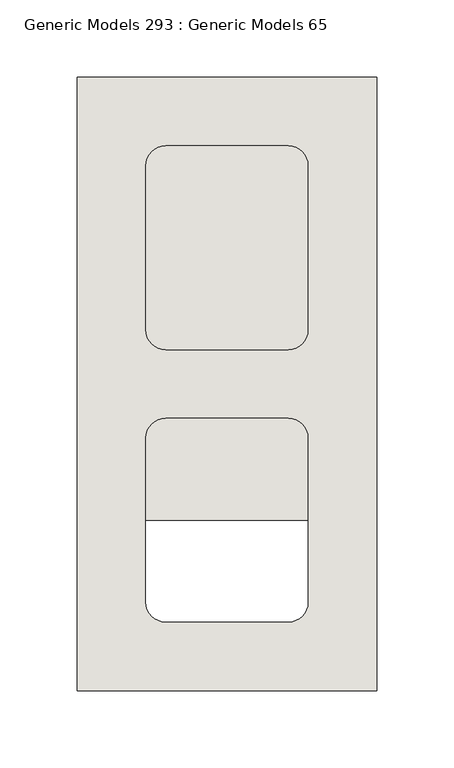
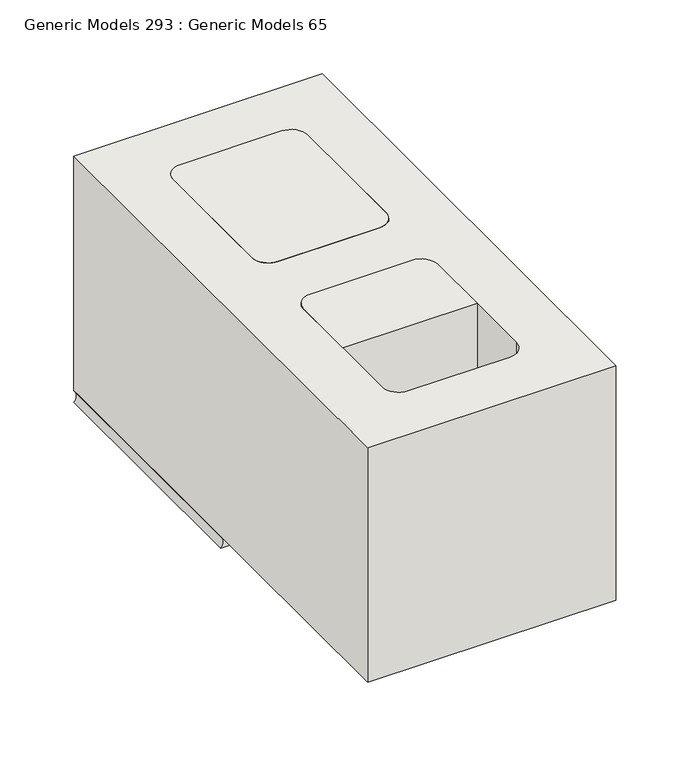
"""IFC4 building model written with IfcOpenShell, lengths in millimetres: wall geometry, Generic Models 293 : Generic Models 65."""

from ifc_helpers import new_model, si_unit, point, frame, frame_2d, origin, place, context, project, spatial, polyline, circle_curve, trimmed, segment, composite_curve, outline, extrude, source, transform, mapped, element, save
from ifc_brep_helpers import plane_surface, revolved_surface, advanced_brep


def generic_models_293_generic_models_65_16f1c2ea(model_context):
    return source(origin(), model_context, "Body", "SolidModel", [
        advanced_brep(
        [(430198.2125, 503.2375, 212.725), (430004.5375, 503.2375, 212.725), (430004.5375, 503.2375, 203.2), (430198.2125, 503.2375, 203.2), (430198.2125, 701.675, 212.725), (430198.2125, 701.675, 203.2), (430004.5375, 701.675, 203.2), (430004.5375, 701.675, 212.725), (430153.7625, 538.1625, 212.725), (430141.0625, 525.4625, 212.725), (430061.6875, 525.4625, 212.725), (430048.9875, 538.1625, 212.725), (430048.9875, 644.525, 212.725), (430061.6875, 657.225, 212.725), (430141.0625, 657.225, 212.725), (430153.7625, 644.525, 212.725), (430141.0625, 525.4625, 203.2), (430153.7625, 538.1625, 203.2), (430061.6875, 525.4625, 203.2), (430048.9875, 538.1625, 203.2), (430048.9875, 644.525, 203.2), (430061.6875, 657.225, 203.2), (430141.0625, 657.225, 203.2), (430153.7625, 644.525, 203.2)],
        [
            (0, 1),
            (1, 2, circle_curve(frame((429999.6545028, 503.2375, 207.9625), z_axis=(0.0, 1.0, 0.0), x_axis=(1.0, 0.0, 0.0)), 6.8209287)),
            (2, 3),
            (3, 0, circle_curve(frame((430203.0954972, 503.2375, 207.9625), z_axis=(0.0, 1.0, 0.0), x_axis=(-1.0, 0.0, 0.0)), 6.8209287)),
            (4, 5, circle_curve(frame((430203.0954972, 701.675, 207.9625), z_axis=(0.0, -1.0, 0.0), x_axis=(-1.0, 0.0, 0.0)), 6.8209287)),
            (5, 6),
            (6, 7, circle_curve(frame((429999.6545028, 701.675, 207.9625), z_axis=(0.0, -1.0, 0.0), x_axis=(1.0, 0.0, 0.0)), 6.8209287)),
            (7, 4),
            (0, 4),
            (7, 1),
            (8, 9, circle_curve(frame((430141.0625, 538.1625, 212.725), z_axis=(0.0, 0.0, -1.0), x_axis=(-1.0, 0.0, 0.0)), 12.7)),
            (9, 10),
            (10, 11, circle_curve(frame((430061.6875, 538.1625, 212.725), z_axis=(0.0, 0.0, -1.0), x_axis=(-1.0, 0.0, 0.0)), 12.7)),
            (11, 12),
            (12, 13, circle_curve(frame((430061.6875, 644.525, 212.725), z_axis=(0.0, 0.0, -1.0), x_axis=(-1.0, 0.0, 0.0)), 12.7)),
            (13, 14),
            (14, 15, circle_curve(frame((430141.0625, 644.525, 212.725), z_axis=(0.0, 0.0, -1.0), x_axis=(-1.0, 0.0, 0.0)), 12.7)),
            (15, 8),
            (16, 9),
            (8, 17),
            (17, 16, circle_curve(frame((430141.0625, 538.1625, 203.2), z_axis=(0.0, 0.0, -1.0), x_axis=(-1.0, 0.0, 0.0)), 12.7)),
            (16, 18),
            (18, 10),
            (18, 19, circle_curve(frame((430061.6875, 538.1625, 203.2), z_axis=(0.0, 0.0, -1.0), x_axis=(-1.0, 0.0, 0.0)), 12.7)),
            (19, 11),
            (19, 20),
            (20, 12),
            (20, 21, circle_curve(frame((430061.6875, 644.525, 203.2), z_axis=(0.0, 0.0, -1.0), x_axis=(-1.0, 0.0, 0.0)), 12.7)),
            (21, 13),
            (21, 22),
            (22, 14),
            (22, 23, circle_curve(frame((430141.0625, 644.525, 203.2), z_axis=(0.0, 0.0, -1.0), x_axis=(-1.0, 0.0, 0.0)), 12.7)),
            (23, 15),
            (23, 17),
            (6, 2),
            (5, 3),
        ],
        [
            plane_surface(frame((430101.375, 503.2375, 213.121875), z_axis=(0.0, -1.0, 0.0), x_axis=(0.0, 0.0, 1.0))),
            plane_surface(frame((430101.375, 701.675, 213.121875), z_axis=(0.0, 1.0, 0.0), x_axis=(0.0, 0.0, 1.0))),
            plane_surface(frame((430198.2125, 503.2375, 212.725), z_axis=(0.0, 0.0, 1.0), x_axis=(0.0, 1.0, 0.0))),
            revolved_surface(polyline([(430128.3625, 538.1625, 212.725), (430128.3625, 538.1625, 203.2)]), (430141.0625, 538.1625, 396.875), (0.0, 0.0, 1.0)),
            plane_surface(frame((430061.6875, 525.4625, 396.875), z_axis=(0.0, 1.0, 0.0), x_axis=(0.0, 0.0, -1.0))),
            revolved_surface(polyline([(430048.9875, 538.1625, 212.725), (430048.9875, 538.1625, 203.2)]), (430061.6875, 538.1625, 396.875), (0.0, 0.0, 1.0)),
            plane_surface(frame((430048.9875, 644.525, 396.875), z_axis=(1.0, 0.0, 0.0), x_axis=(0.0, 0.0, -1.0))),
            revolved_surface(polyline([(430048.9875, 644.525, 212.725), (430048.9875, 644.525, 203.2)]), (430061.6875, 644.525, 396.875), (0.0, 0.0, 1.0)),
            plane_surface(frame((430141.0625, 657.225, 396.875), z_axis=(0.0, -1.0, 0.0), x_axis=(0.0, 0.0, -1.0))),
            revolved_surface(polyline([(430128.3625, 644.525, 212.725), (430128.3625, 644.525, 203.2)]), (430141.0625, 644.525, 396.875), (0.0, 0.0, 1.0)),
            plane_surface(frame((430153.7625, 538.1625, 396.875), z_axis=(-1.0, 0.0, 0.0), x_axis=(0.0, 0.0, -1.0))),
            revolved_surface(polyline([(430006.4754315, 701.675, 207.9625), (430006.4754315, 503.2375, 207.9625)]), (429999.6545028, 503.2375, 207.9625), (0.0, 1.0, 0.0)),
            plane_surface(frame((430004.5375, 503.2375, 203.2), z_axis=(0.0, 0.0, -1.0), x_axis=(0.0, 1.0, 0.0))),
            revolved_surface(polyline([(430196.2745685, 701.675, 207.9625), (430196.2745685, 503.2375, 207.9625)]), (430203.0954972, 503.2375, 207.9625), (0.0, 1.0, 0.0)),
        ],
        [
            (0, [[1, 2, 3, 4]]),
            (1, [[5, 6, 7, 8]]),
            (2, [[-1, 9, -8, 10], [11, 12, 13, 14, 15, 16, 17, 18]]),
            (3, [[19, -11, 20, 21]]),
            (4, [[-19, 22, 23, -12]]),
            (5, [[-23, 24, 25, -13]]),
            (6, [[-25, 26, 27, -14]]),
            (7, [[-27, 28, 29, -15]]),
            (8, [[-29, 30, 31, -16]]),
            (9, [[-31, 32, 33, -17]]),
            (10, [[-33, 34, -20, -18]]),
            (11, [[-2, -10, -7, 35]]),
            (12, [[-3, -35, -6, 36], [-21, -34, -32, -30, -28, -26, -24, -22]]),
            (13, [[-4, -36, -5, -9]]),
        ],
    ),
        extrude(outline(composite_curve([segment(trimmed(circle_curve(frame_2d((430141.0625, 538.1625)), 12.7), [point((430153.7625, 538.1625))], [point((430141.0625, 525.4625))], False, "CARTESIAN"), True, "CONTINUOUS"), segment(polyline([(430141.0625, 525.4625), (430061.6875, 525.4625)]), True, "CONTINUOUS"), segment(trimmed(circle_curve(frame_2d((430061.6875, 538.1625)), 12.7), [point((430061.6875, 525.4625))], [point((430048.9875, 538.1625))], False, "CARTESIAN"), True, "CONTINUOUS"), segment(polyline([(430048.9875, 538.1625), (430048.9875, 644.525)]), True, "CONTINUOUS"), segment(trimmed(circle_curve(frame_2d((430061.6875, 644.525)), 12.7), [point((430048.9875, 644.525))], [point((430061.6875, 657.225))], False, "CARTESIAN"), True, "CONTINUOUS"), segment(polyline([(430061.6875, 657.225), (430141.0625, 657.225)]), True, "CONTINUOUS"), segment(trimmed(circle_curve(frame_2d((430141.0625, 644.525)), 12.7), [point((430141.0625, 657.225))], [point((430153.7625, 644.525))], False, "CARTESIAN"), True, "CONTINUOUS"), segment(polyline([(430153.7625, 644.525), (430153.7625, 538.1625)]), True, "CONTINUOUS")], self_intersect=False)), frame((0.0, 0.0, 203.2), z_axis=(0.0, 0.0, 1.0), x_axis=(1.0, 0.0, 0.0)), (0.0, 0.0, 1.0), 203.2),
        extrude(outline(composite_curve([segment(trimmed(circle_curve(frame_2d((430061.6875, 468.3125)), 12.7), [point((430048.9875, 468.3125))], [point((430061.6875, 481.0125))], False, "CARTESIAN"), True, "CONTINUOUS"), segment(polyline([(430061.6875, 481.0125), (430141.0625, 481.0125)]), True, "CONTINUOUS"), segment(trimmed(circle_curve(frame_2d((430141.0625, 468.3125)), 12.7), [point((430141.0625, 481.0125))], [point((430153.7625, 468.3125))], False, "CARTESIAN"), True, "CONTINUOUS"), segment(polyline([(430153.7625, 468.3125), (430153.7625, 415.13125), (430048.9875, 415.13125), (430048.9875, 468.3125)]), True, "CONTINUOUS")], self_intersect=False)), frame((0.0, 0.0, 203.2), z_axis=(0.0, 0.0, 1.0), x_axis=(1.0, 0.0, 0.0)), (0.0, 0.0, 1.0), 203.2),
        extrude(outline(polyline([(430198.2125, 304.8), (430004.5375, 304.8), (430004.5375, 701.675), (430198.2125, 701.675), (430198.2125, 304.8)]), holes=[composite_curve([segment(polyline([(430153.7625, 538.1625), (430153.7625, 644.525)]), True, "CONTINUOUS"), segment(trimmed(circle_curve(frame_2d((430141.0625, 644.525)), 12.7), [point((430153.7625, 644.525))], [point((430141.0625, 657.225))], True, "CARTESIAN"), True, "CONTINUOUS"), segment(polyline([(430141.0625, 657.225), (430061.6875, 657.225)]), True, "CONTINUOUS"), segment(trimmed(circle_curve(frame_2d((430061.6875, 644.525)), 12.7), [point((430061.6875, 657.225))], [point((430048.9875, 644.525))], True, "CARTESIAN"), True, "CONTINUOUS"), segment(polyline([(430048.9875, 644.525), (430048.9875, 538.1625)]), True, "CONTINUOUS"), segment(trimmed(circle_curve(frame_2d((430061.6875, 538.1625)), 12.7), [point((430048.9875, 538.1625))], [point((430061.6875, 525.4625))], True, "CARTESIAN"), True, "CONTINUOUS"), segment(polyline([(430061.6875, 525.4625), (430141.0625, 525.4625)]), True, "CONTINUOUS"), segment(trimmed(circle_curve(frame_2d((430141.0625, 538.1625)), 12.7), [point((430141.0625, 525.4625))], [point((430153.7625, 538.1625))], True, "CARTESIAN"), True, "CONTINUOUS")], self_intersect=False), composite_curve([segment(polyline([(430048.9875, 468.3125), (430048.9875, 361.95)]), True, "CONTINUOUS"), segment(trimmed(circle_curve(frame_2d((430061.6875, 361.95)), 12.7), [point((430048.9875, 361.95))], [point((430061.6875, 349.25))], True, "CARTESIAN"), True, "CONTINUOUS"), segment(polyline([(430061.6875, 349.25), (430141.0625, 349.25)]), True, "CONTINUOUS"), segment(trimmed(circle_curve(frame_2d((430141.0625, 361.95)), 12.7), [point((430141.0625, 349.25))], [point((430153.7625, 361.95))], True, "CARTESIAN"), True, "CONTINUOUS"), segment(polyline([(430153.7625, 361.95), (430153.7625, 468.3125)]), True, "CONTINUOUS"), segment(trimmed(circle_curve(frame_2d((430141.0625, 468.3125)), 12.7), [point((430153.7625, 468.3125))], [point((430141.0625, 481.0125))], True, "CARTESIAN"), True, "CONTINUOUS"), segment(polyline([(430141.0625, 481.0125), (430061.6875, 481.0125)]), True, "CONTINUOUS"), segment(trimmed(circle_curve(frame_2d((430061.6875, 468.3125)), 12.7), [point((430061.6875, 481.0125))], [point((430048.9875, 468.3125))], True, "CARTESIAN"), True, "CONTINUOUS")], self_intersect=False)]), frame((0.0, 0.0, 212.725), z_axis=(0.0, 0.0, 1.0), x_axis=(1.0, 0.0, 0.0)), (0.0, 0.0, 1.0), 193.675),
    ])


if __name__ == "__main__":
    model = new_model("IFC4")
    model_context = context("Model", 3, world=origin())
    ifc_project = project(units=[si_unit("LENGTHUNIT", "METRE", prefix="MILLI")], contexts=[model_context])
    site = spatial("IfcSite", under=ifc_project)
    building = spatial("IfcBuilding", under=site)
    placement = place(None, origin())
    generic_models_293_generic_models_65_shape = generic_models_293_generic_models_65_16f1c2ea(model_context)
    element("IfcWall", 1, ObjectType="Generic Models 293 : Generic Models 65", at=placement, inside=building, context=model_context, shape_type="MappedRepresentation", body=[
        mapped(generic_models_293_generic_models_65_shape, transform((0.0, 0.0, 0.0), x_axis=(1.0, 0.0, 0.0), y_axis=(0.0, 1.0, 0.0), z_axis=(0.0, 0.0, 1.0))),
    ])
    save(model, "model.ifc")

# Revit data of these elements
# Element 1 (IfcWall, "Generic Models 293 : Generic Models 65")
#   Materials on its faces: "CMU (SEE 'WALL TAG' FOR SIZE)", "FILL CORE IF APPLICABLE - SEE STRUCTURAL DWGS FOR DETAILS", "MORTAR JOINT"
# Materials
#   "CMU (SEE 'WALL TAG' FOR SIZE)": class "Masonry", colour RGB 203 203 199, transparency 0, Description = "Concrete masonry units", Cost = 0
#   "FILL CORE IF APPLICABLE - SEE STRUCTURAL DWGS FOR DETAILS": class "Generic", colour RGB 170 170 170, transparency 0, Cost = 0
#   "MORTAR JOINT": class "Generic", colour RGB 120 120 120, transparency 0, Cost = 0
